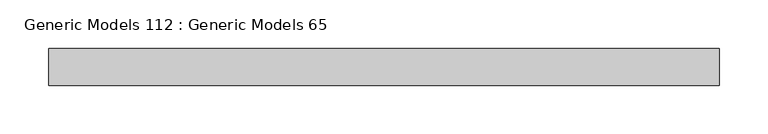
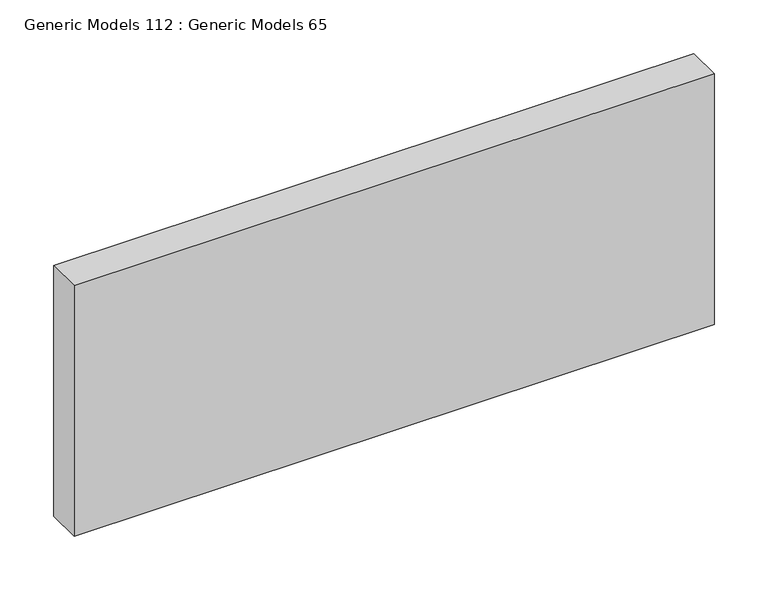
"""IFC4 building model written with IfcOpenShell, lengths in millimetres: proxy geometry, Generic Models 112 : Generic Models 65."""

from ifc_helpers import new_model, si_unit, frame, origin, place, context, project, spatial, polyline, outline, extrude, source, transform, mapped, element, save


def generic_models_112_generic_models_65_d168d7b0(model_context):
    return source(origin(), model_context, "Body", "SweptSolid", [
        extrude(outline(polyline([(50952.4, 592.1375), (50952.4, 630.2375), (51642.1451407, 630.2375), (51642.1451407, 592.1375), (50952.4, 592.1375)])), frame((0.0, 0.0, 5222.478125), z_axis=(0.0, 0.0, 1.0), x_axis=(1.0, 0.0, 0.0)), (0.0, 0.0, 1.0), 285.75),
    ])


if __name__ == "__main__":
    model = new_model("IFC4")
    model_context = context("Model", 3, world=origin())
    ifc_project = project(units=[si_unit("LENGTHUNIT", "METRE", prefix="MILLI")], contexts=[model_context])
    site = spatial("IfcSite", under=ifc_project)
    building = spatial("IfcBuilding", under=site)
    placement = place(None, origin())
    generic_models_112_generic_models_65_shape = generic_models_112_generic_models_65_d168d7b0(model_context)
    element("IfcBuildingElementProxy", 1, Name="Generic Models 112 : Generic Models 65", ObjectType="Generic Models 112 : Generic Models 65", at=placement, inside=building, context=model_context, shape_type="MappedRepresentation", body=[
        mapped(generic_models_112_generic_models_65_shape, transform((0.0, 0.0, 0.0), x_axis=(1.0, 0.0, 0.0), y_axis=(0.0, 1.0, 0.0), z_axis=(0.0, 0.0, 1.0))),
    ])
    save(model, "model.ifc")

# Revit data of these elements
# Element 1 (IfcBuildingElementProxy, "Generic Models 112 : Generic Models 65")
#   Materials on its faces: "WOOD JOIST AS SPECIFIED"
# Materials
#   "WOOD JOIST AS SPECIFIED": class "Wood", colour RGB 234 198 147, transparency 0, Description = "Pinus Echinata", Cost = 0
